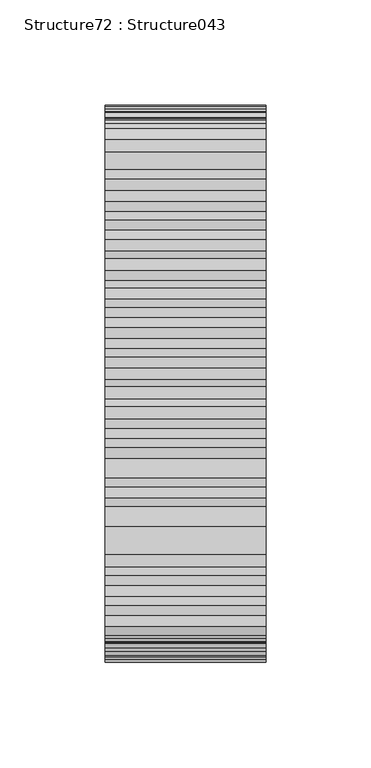
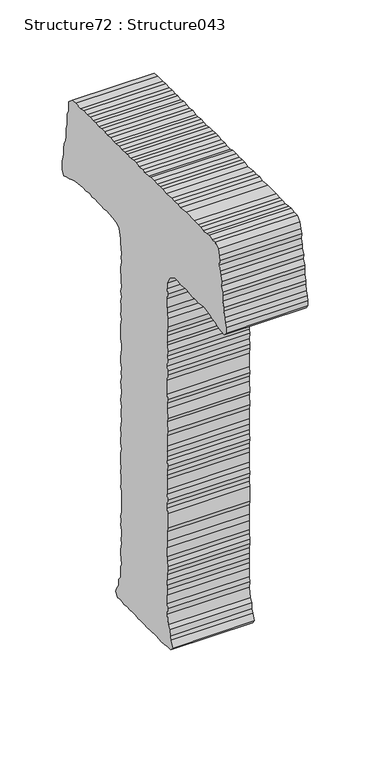
"""IFC4 building model written with IfcOpenShell, lengths in millimetres: proxy geometry, Structure72 : Structure043."""

from ifc_helpers import new_model, si_unit, frame, origin, place, context, project, spatial, polyline, outline, extrude, source, transform, mapped, element, save


def structure72_structure043_2b378016(model_context):
    return source(origin(), model_context, "Body", "SweptSolid", [
        extrude(outline(polyline([(277031.5025635, 3992.8375436), (277035.602328, 3996.9645864), (277040.8622215, 3996.390138), (277045.5653173, 3997.5486624), (277049.6650818, 3996.9645864), (277054.9249753, 3996.390138), (277059.6280711, 3996.9645864), (277063.7053711, 3996.9645864), (277069.5669913, 3997.5486624), (277083.0729474, 3997.5486624), (277092.4326054, 3996.390138), (277096.5339745, 3997.5486624), (277101.7922634, 3996.9645864), (277105.916097, 3997.5486624), (277115.275755, 3996.390138), (277120.558113, 3997.5486624), (277124.6578775, 3997.5486624), (277129.3385088, 3996.9645864), (277134.0416046, 3997.5486624), (277139.8791557, 3997.5486624), (277143.4237271, 3996.390138), (277149.2628828, 3996.390138), (277152.7833851, 3996.9645864), (277158.0657431, 3996.9645864), (277163.3256366, 3997.5486624), (277167.4254011, 3997.5486624), (277172.1284969, 3996.9645864), (277177.3867858, 3997.5486624), (277182.0674171, 3996.390138), (277186.7705129, 3996.390138), (277190.8702774, 3996.9645864), (277196.1526354, 3996.390138), (277199.6506732, 3996.390138), (277204.3313045, 3997.5486624), (277210.2153892, 3996.390138), (277213.713427, 3997.5486624), (277218.995785, 3997.5486624), (277223.6764163, 3996.390138), (277228.355443, 3997.5486624), (277232.4792766, 3996.9645864), (277237.1583033, 3997.5486624), (277242.4181968, 3996.9645864), (277247.7005548, 3997.5486624), (277252.3811861, 3996.9645864), (277260.5823197, 3996.9645864), (277266.4423353, 3996.390138), (277271.7246933, 3991.6806238), (277271.7246933, 3988.1633307), (277271.7246933, 3982.8793681), (277274.0642067, 3978.2035506), (277274.0642067, 3974.1214368), (277274.0642067, 3968.2357475), (277275.8260624, 3963.5615346), (277275.8260624, 3958.8776941), (277276.4053246, 3954.7506513), (277277.0070513, 3950.6765605), (277279.3241002, 3946.5511223), (277279.9258269, 3941.2912288), (277279.9258269, 3936.0345445), (277281.0843513, 3931.9058971), (277282.2669449, 3927.2332888), (277282.2669449, 3921.9733953), (277282.8462071, 3918.4480792), (277279.9258269, 3914.3499193), (277274.6450735, 3916.0909152), (277271.1454311, 3916.6653636), (277266.4423353, 3918.4480792), (277261.7633086, 3919.6066036), (277248.3022815, 3921.3748778), (277244.1784479, 3920.7908018), (277238.3184323, 3921.9733953), (277234.2170632, 3920.7908018), (277230.1172987, 3921.9733953), (277224.8574052, 3920.7908018), (277220.1543094, 3921.3748778), (277214.8944159, 3920.7908018), (277210.2153892, 3921.3748778), (277206.6932823, 3921.3748778), (277200.8332667, 3920.7908018), (277193.7906576, 3919.0321552), (277190.2685507, 3916.6653636), (277187.9515018, 3907.888177), (277187.9515018, 3903.7884125), (277187.3497751, 3899.1061766), (277186.7705129, 3893.822214), (277187.3497751, 3890.320967), (277186.7705129, 3885.6210804), (277187.9515018, 3879.7610648), (277187.9515018, 3876.263027), (277187.3497751, 3870.9790644), (277187.3497751, 3866.3032469), (277186.7705129, 3861.6178018), (277187.9515018, 3856.3161885), (277186.7705129, 3851.6612309), (277187.9515018, 3846.9757858), (277187.3497751, 3842.2758992), (277187.3497751, 3837.6000817), (277187.9515018, 3833.4730389), (277186.7705129, 3829.374879), (277187.9515018, 3823.5341187), (277187.9515018, 3809.4729695), (277186.7705129, 3804.7730829), (277186.7705129, 3800.6717138), (277187.3497751, 3795.960595), (277187.9515018, 3791.8865042), (277187.9515018, 3786.6298199), (277186.7705129, 3781.3282066), (277187.3497751, 3776.6427615), (277186.7705129, 3772.5606477), (277187.9515018, 3767.2590344), (277187.3497751, 3763.759392), (277186.7705129, 3757.8753073), (277187.3497751, 3753.2171405), (277187.9515018, 3749.701452), (277186.7705129, 3743.2332913), (277187.3497751, 3739.7416719), (277187.3497751, 3734.47536), (277186.7705129, 3730.3563402), (277187.9515018, 3720.9726131), (277187.3497751, 3715.7143242), (277187.9515018, 3711.0304837), (277187.9515018, 3706.9130685), (277186.7705129, 3702.229228), (277187.9515018, 3696.9709391), (277187.9515018, 3687.0127636), (277187.3497751, 3683.4858429), (277187.9515018, 3678.81163), (277187.3497751, 3674.1277895), (277187.3497751, 3668.2437048), (277187.9515018, 3663.5598643), (277186.7705129, 3660.0682449), (277186.7705129, 3640.114988), (277187.9515018, 3635.4407751), (277187.3497751, 3630.7392839), (277187.9515018, 3626.6571701), (277186.7705129, 3621.9813526), (277186.7705129, 3617.8559144), (277187.3497751, 3612.0135494), (277186.7705129, 3608.4705827), (277187.9515018, 3602.6298224), (277187.9515018, 3598.5284533), (277187.3497751, 3593.2541183), (277186.7705129, 3588.5702778), (277187.9515018, 3585.0706354), (277188.530764, 3574.5107332), (277191.4495396, 3570.9854171), (277191.4495396, 3565.1254015), (277194.3923843, 3560.441561), (277196.1526354, 3556.3417965), (277193.2113953, 3551.6675836), (277188.530764, 3552.242032), (277182.6466793, 3551.0658569), (277177.9676526, 3552.242032), (277173.888748, 3551.6675836), (277168.60639, 3552.242032), (277163.9273633, 3552.242032), (277159.8035297, 3551.0658569), (277155.7037653, 3551.6675836), (277150.4438717, 3551.6675836), (277145.7407759, 3551.0658569), (277140.4808824, 3551.6675836), (277131.0987599, 3551.6675836), (277126.4197332, 3551.0658569), (277122.8976263, 3551.0658569), (277117.0360061, 3551.6675836), (277112.3569794, 3552.242032), (277107.6538836, 3552.242032), (277104.7351081, 3555.7416744), (277107.6538836, 3561.6257591), (277108.8348725, 3565.1254015), (277109.4141348, 3570.9854171), (277111.7777172, 3574.5107332), (277112.9362416, 3583.8864372), (277112.3569794, 3589.7544759), (277112.9362416, 3594.4286888), (277112.9362416, 3602.6298224), (277113.5379683, 3607.8961343), (277112.9362416, 3612.5976255), (277112.9362416, 3617.2718384), (277113.5379683, 3622.555801), (277112.3569794, 3627.2396415), (277112.3569794, 3631.3410106), (277113.5379683, 3636.0408972), (277112.9362416, 3640.7167147), (277112.9362416, 3649.5003197), (277113.5379683, 3655.3587307), (277113.5379683, 3664.7440624), (277112.3569794, 3668.8261762), (277112.3569794, 3683.4858429), (277112.9362416, 3688.1873341), (277112.9362416, 3692.2710525), (277112.3569794, 3696.3884676), (277112.9362416, 3702.229228), (277113.5379683, 3706.3289925), (277113.5379683, 3716.2887726), (277112.9362416, 3720.9726131), (277113.5379683, 3725.0996559), (277112.3569794, 3729.7738688), (277112.9362416, 3735.0578314), (277113.5379683, 3738.5574738), (277112.9362416, 3744.4158848), (277113.5379683, 3749.117376), (277113.5379683, 3759.0595054), (277112.3569794, 3763.759392), (277113.5379683, 3773.11905), (277112.3569794, 3776.6427615), (277113.5379683, 3786.0280932), (277113.5379683, 3791.3056374), (277112.3569794, 3795.4037973), (277112.9362416, 3800.6717138), (277112.9362416, 3814.148787), (277112.3569794, 3819.4150989), (277112.3569794, 3823.5341187), (277112.9362416, 3828.2163546), (277112.3569794, 3834.0474873), (277113.5379683, 3837.6000817), (277112.3569794, 3842.8583706), (277113.5379683, 3848.1166595), (277112.9362416, 3851.6612309), (277113.5379683, 3857.5019912), (277113.5379683, 3861.0192843), (277112.3569794, 3866.8776953), (277112.3569794, 3875.0772243), (277113.5379683, 3879.7610648), (277112.9362416, 3885.6210804), (277112.9362416, 3894.4030808), (277112.3569794, 3899.1061766), (277112.9362416, 3904.3901392), (277113.5379683, 3909.0627475), (277109.4141348, 3916.6653636), (277101.2130012, 3921.9733953), (277096.5339745, 3921.9733953), (277090.6723543, 3921.3748778), (277087.1502474, 3921.9733953), (277081.8919585, 3921.9733953), (277077.1888627, 3920.7908018), (277073.0874936, 3920.7908018), (277067.2499424, 3921.3748778), (277062.5468467, 3920.7908018), (277058.4454776, 3921.3748778), (277053.1871886, 3921.9733953), (277044.3843284, 3919.6066036), (277040.8622215, 3918.4480792), (277036.1815902, 3917.8479571), (277032.0818257, 3916.0909152), (277027.4011944, 3914.9307861), (277021.5395742, 3914.3499193), (277018.5983341, 3917.8479571), (277018.5983341, 3923.1319197), (277019.779323, 3927.2332888), (277020.9603119, 3931.3346579), (277022.120441, 3937.1930689), (277022.120441, 3940.718385), (277023.8806921, 3945.9766739), (277023.8806921, 3951.2606365), (277023.8806921, 3954.7506513), (277026.2202055, 3959.4617701), (277025.6184788, 3964.1343784), (277027.4011944, 3969.418341), (277027.9804566, 3972.9372387), (277029.1614455, 3978.2035506), (277028.5597188, 3982.8793681), (277029.7423123, 3987.0048063), (277031.5025635, 3992.8375436)])), frame((-59031.6926606, 0.0, 0.0), z_axis=(1.0, 0.0, 0.0), x_axis=(0.0, 1.0, 0.0)), (0.0, 0.0, 1.0), 76.2),
    ])


if __name__ == "__main__":
    model = new_model("IFC4")
    model_context = context("Model", 3, world=origin())
    ifc_project = project(units=[si_unit("LENGTHUNIT", "METRE", prefix="MILLI")], contexts=[model_context])
    site = spatial("IfcSite", under=ifc_project)
    building = spatial("IfcBuilding", under=site)
    placement = place(None, origin())
    structure72_structure043_shape = structure72_structure043_2b378016(model_context)
    element("IfcBuildingElementProxy", 1, Name="Structure72 : Structure043", ObjectType="Structure72 : Structure043", at=placement, inside=building, context=model_context, shape_type="MappedRepresentation", body=[
        mapped(structure72_structure043_shape, transform((0.0, 0.0, 0.0), x_axis=(1.0, 0.0, 0.0), y_axis=(0.0, 1.0, 0.0), z_axis=(0.0, 0.0, 1.0))),
    ])
    save(model, "model.ifc")

# Revit data of these elements
# Type "Structure72 : Structure043"
#   NameOverride = "Structure043"
# Element 1 (IfcBuildingElementProxy, "Structure72 : Structure043")
#   Materials on its faces: "BRUSHED ALUM. LETTERING"
# Materials
#   "BRUSHED ALUM. LETTERING": class "Unassigned", colour RGB 169 181 186, transparency 0, Cost = 0
